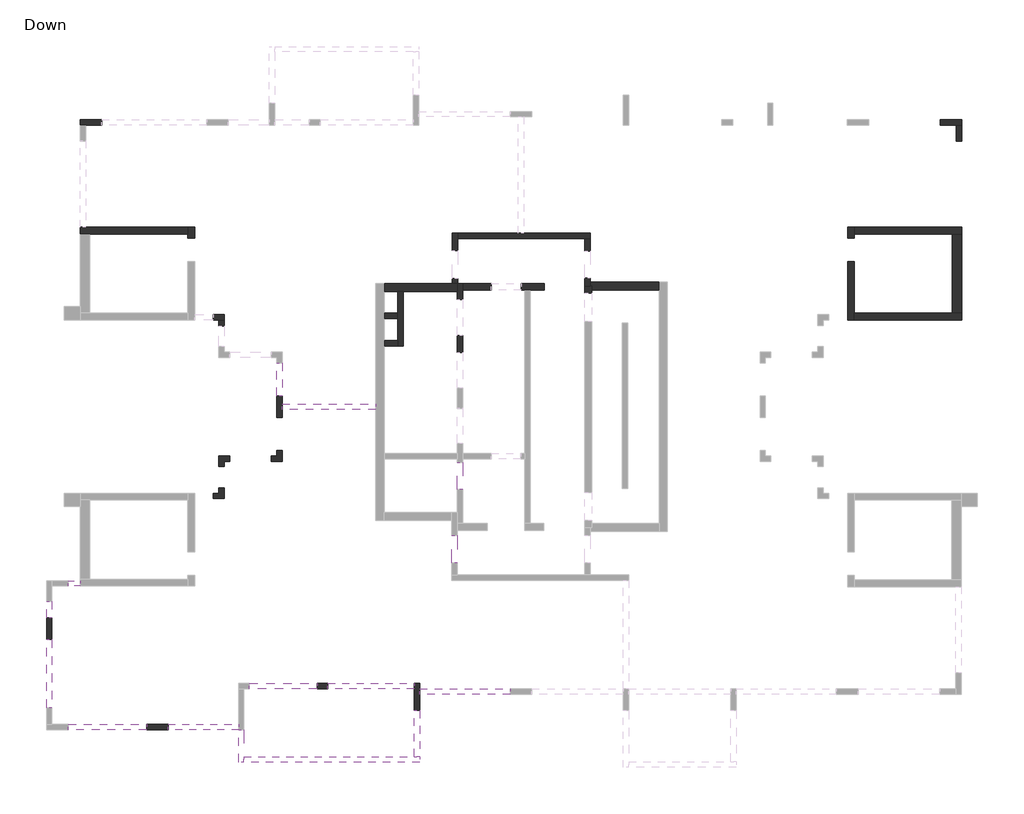
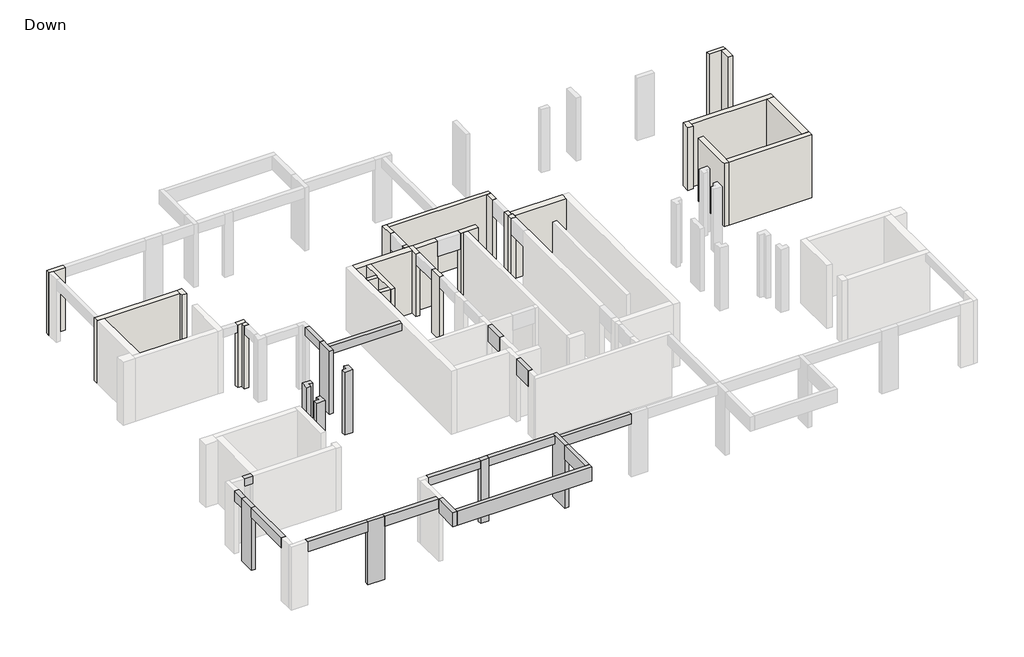
# One storey, part 2 of 3: 27 walls, 15 beams, 8 columns.
# Revit data of these elements (continued)
# Element 40 (IfcWall, "25") (continued)
#   Comments = ""
#   Mark = "W61"
#   SOFiSTiK_EdgeZones = "W63"
#   SOFiSTiK_AMG_Comments = ""
#   Top Offset = 0 cm
#   Base Offset = 0 cm
#   wall height = 320 cm
#   SOFiSTiK_AMG_Scheduled = yes
#   SOFiSTiK_AMG_Adjusted = yes
#   Phase Created = New Construction
#   Base Constraint = Down
#   Top Constraint = Typical Floor
#   Materials on its faces: "Concrete"
# Element 41 (IfcWall, "25")
#   Comments = ""
#   Mark = "W64"
#   SOFiSTiK_EdgeZones = "W66"
#   SOFiSTiK_AMG_Comments = ""
#   Top Offset = 0 cm
#   Base Offset = 0 cm
#   wall height = 320 cm
#   SOFiSTiK_AMG_Scheduled = yes
#   SOFiSTiK_AMG_Adjusted = yes
#   Phase Created = New Construction
#   Base Constraint = Down
#   Top Constraint = Typical Floor
#   Materials on its faces: "Concrete"
# Element 42 (IfcWall, "25")
#   Comments = ""
#   Mark = "W65"
#   SOFiSTiK_EdgeZones = "W67"
#   SOFiSTiK_AMG_Comments = ""
#   Top Offset = 0 cm
#   Base Offset = 0 cm
#   wall height = 320 cm
#   SOFiSTiK_AMG_Scheduled = yes
#   SOFiSTiK_AMG_Adjusted = yes
#   Phase Created = New Construction
#   Base Constraint = Down
#   Top Constraint = Typical Floor
#   Materials on its faces: "Concrete"
# Element 43 (IfcWall, "25")
#   Comments = ""
#   Mark = "W66"
#   SOFiSTiK_EdgeZones = "W68"
#   SOFiSTiK_AMG_Comments = ""
#   Top Offset = 0 cm
#   Base Offset = 0 cm
#   wall height = 320 cm
#   SOFiSTiK_AMG_Scheduled = yes
#   SOFiSTiK_AMG_Adjusted = yes
#   Phase Created = New Construction
#   Base Constraint = Down
#   Top Constraint = Typical Floor
#   Materials on its faces: "Concrete"
# Element 44 (IfcWall, "25")
#   Comments = ""
#   Mark = "W67"
#   SOFiSTiK_EdgeZones = "W69"
#   SOFiSTiK_AMG_Comments = ""
#   Top Offset = 0 cm
#   Base Offset = 0 cm
#   wall height = 320 cm
#   SOFiSTiK_AMG_Scheduled = yes
#   SOFiSTiK_AMG_Adjusted = yes
#   Phase Created = New Construction
#   Base Constraint = Down
#   Top Constraint = Typical Floor
#   Materials on its faces: "Concrete"
# Element 45 (IfcWall, "25")
#   Comments = ""
#   Mark = "W68"
#   SOFiSTiK_EdgeZones = "W70"
#   SOFiSTiK_AMG_Comments = ""
#   Top Offset = 0 cm
#   Base Offset = 0 cm
#   wall height = 320 cm
#   SOFiSTiK_AMG_Scheduled = yes
#   SOFiSTiK_AMG_Adjusted = yes
#   Phase Created = New Construction
#   Base Constraint = Down
#   Top Constraint = Typical Floor
#   Materials on its faces: "Concrete"
# Element 46 (IfcWall, "25")
#   Comments = ""
#   Mark = "W69"
#   SOFiSTiK_EdgeZones = "W71"
#   SOFiSTiK_AMG_Comments = ""
#   Top Offset = 0 cm
#   Base Offset = 0 cm
#   wall height = 320 cm
#   SOFiSTiK_AMG_Scheduled = yes
#   SOFiSTiK_AMG_Adjusted = yes
#   Phase Created = New Construction
#   Base Constraint = Down
#   Top Constraint = Typical Floor
#   Materials on its faces: "Concrete"
# Element 47 (IfcWall, "25")
#   Comments = ""
#   Mark = "W70"
#   SOFiSTiK_EdgeZones = "W72"
#   SOFiSTiK_AMG_Comments = ""
#   Top Offset = 0 cm
#   Base Offset = 0 cm
#   wall height = 320 cm
#   SOFiSTiK_AMG_Scheduled = yes
#   SOFiSTiK_AMG_Adjusted = yes
#   Phase Created = New Construction
#   Base Constraint = Down
#   Top Constraint = Typical Floor
#   Materials on its faces: "Concrete"
# Element 48 (IfcWall, "30")
#   Comments = ""
#   Mark = "W92"
#   SOFiSTiK_EdgeZones = "W94"
#   SOFiSTiK_AMG_Comments = ""
#   Top Offset = 0 cm
#   Base Offset = 0 cm
#   wall height = 320 cm
#   SOFiSTiK_AMG_Scheduled = yes
#   SOFiSTiK_AMG_Adjusted = yes
#   Phase Created = New Construction
#   Base Constraint = Down
#   Top Constraint = Typical Floor
#   Materials on its faces: "Concrete"
# Element 49 (IfcWall, "30")
#   Comments = ""
#   Mark = "W95"
#   SOFiSTiK_EdgeZones = "W97"
#   SOFiSTiK_AMG_Comments = ""
#   Top Offset = 0 cm
#   Base Offset = 0 cm
#   wall height = 320 cm
#   SOFiSTiK_AMG_Scheduled = yes
#   SOFiSTiK_AMG_Adjusted = yes
#   Phase Created = New Construction
#   Base Constraint = Down
#   Top Constraint = Typical Floor
#   Materials on its faces: "Concrete"
# Element 50 (IfcWall, "35")
#   Comments = ""
#   Mark = "W84"
#   SOFiSTiK_EdgeZones = "W86"
#   SOFiSTiK_AMG_Comments = ""
#   Top Offset = 0 cm
#   Base Offset = 0 cm
#   wall height = 320 cm
#   SOFiSTiK_AMG_Scheduled = yes
#   SOFiSTiK_AMG_Adjusted = yes
#   Phase Created = New Construction
#   Base Constraint = Down
#   Top Constraint = Typical Floor
#   Materials on its faces: "Concrete"
# Materials
#   "Concrete": class "Concrete", colour RGB 192 192 192, transparency 0, Keynote = "01000", Description = "Cast-in-place concrete", Cost = 0
#   "Concrete, Cast-in-Place gray": class "Concrete", colour RGB 192 192 192, transparency 0, Description = "Cast-in-place concrete", Cost = 0
